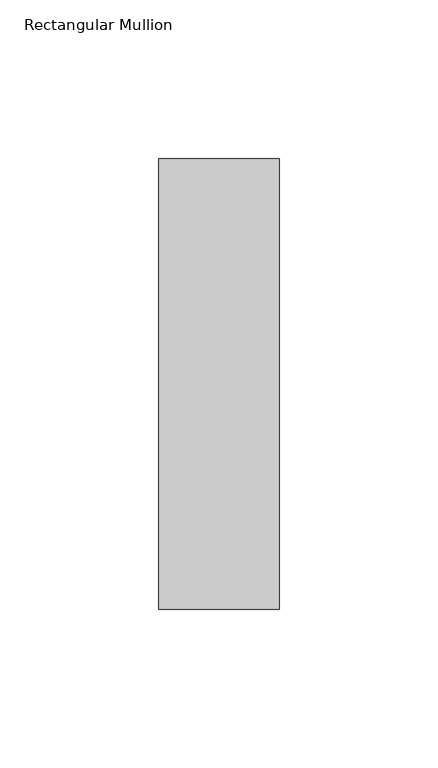
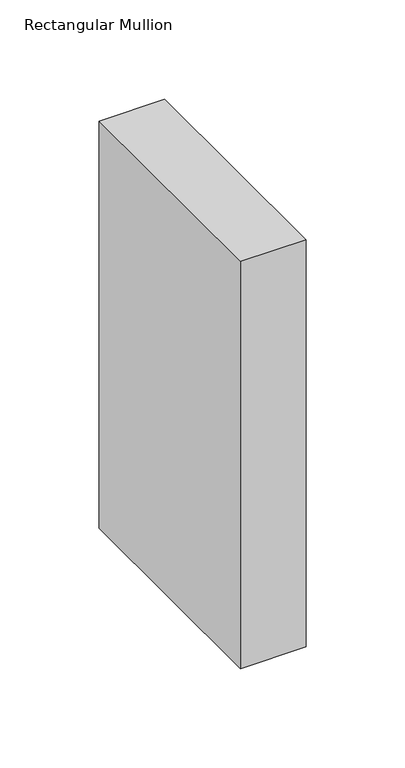
"""IFC4 building model written with IfcOpenShell, lengths in millimetres: member geometry, Rectangular Mullion : NLRS_21_CWM_hsb-regel 38x142_gen_rsf."""

from ifc_helpers import new_model, si_unit, frame, origin, place, context, project, spatial, polyline, outline, extrude, source, transform, mapped, element, save


def rectangular_mullion_597468ba(model_context):
    return source(origin(), model_context, "Body", "SweptSolid", [
        extrude(outline(polyline([(0.0, -71.0), (-38.0, -71.0), (-38.0, 71.0), (0.0, 71.0), (0.0, -71.0)])), frame((0.0, 0.0, -250.0000003), z_axis=(0.0, 0.0, 1.0), x_axis=(1.0, 0.0, 0.0)), (0.0, 0.0, 1.0), 250.0000003),
    ])


if __name__ == "__main__":
    model = new_model("IFC4")
    model_context = context("Model", 3, world=origin())
    ifc_project = project(units=[si_unit("LENGTHUNIT", "METRE", prefix="MILLI")], contexts=[model_context])
    site = spatial("IfcSite", under=ifc_project)
    building = spatial("IfcBuilding", under=site)
    placement = place(None, origin())
    rectangular_mullion_shape = rectangular_mullion_597468ba(model_context)
    element("IfcMember", 1, ObjectType="Rectangular Mullion : NLRS_21_CWM_hsb-regel 38x142_gen_rsf", at=placement, inside=building, context=model_context, shape_type="MappedRepresentation", body=[
        mapped(rectangular_mullion_shape, transform((0.0, 0.0, 0.0), x_axis=(1.0, 0.0, 0.0), y_axis=(0.0, 1.0, 0.0), z_axis=(0.0, 0.0, 1.0))),
    ])
    save(model, "model.ifc")

# Revit data of these elements
# Type "Rectangular Mullion : NLRS_21_CWM_hsb-regel 38x142_gen_rsf"
#   Export Type to IFC As = "IfcWall"
#   Type IfcGUID = "07M7mRoiH1CR8m_RSKIwpF"
#   Assembly Code = "21.10"
#   built-in parameter 1007322 = 0.465879 (stored number, unit not read)
#   built-in parameter 1007321 = 0.062336 (stored number, unit not read)
#   built-in parameter 1007320 = 0.062336 (stored number, unit not read)
# Element 1 (IfcMember, "Rectangular Mullion : NLRS_21_CWM_hsb-regel 38x142_gen_rsf")
#   Materials on its faces: "NLRS_i2_hout naaldhout vuren_gen_rsf"
# Materials
#   "NLRS_i2_hout naaldhout vuren_gen_rsf": class "I - Hout", colour RGB 234 199 147, transparency 0, Keynote = "i2", Manufacturer = "Revit Standards Foundation", URL = "www.revitstandards.org", Description = "hout vuren", Cost = 0
